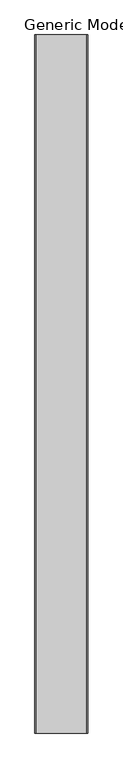
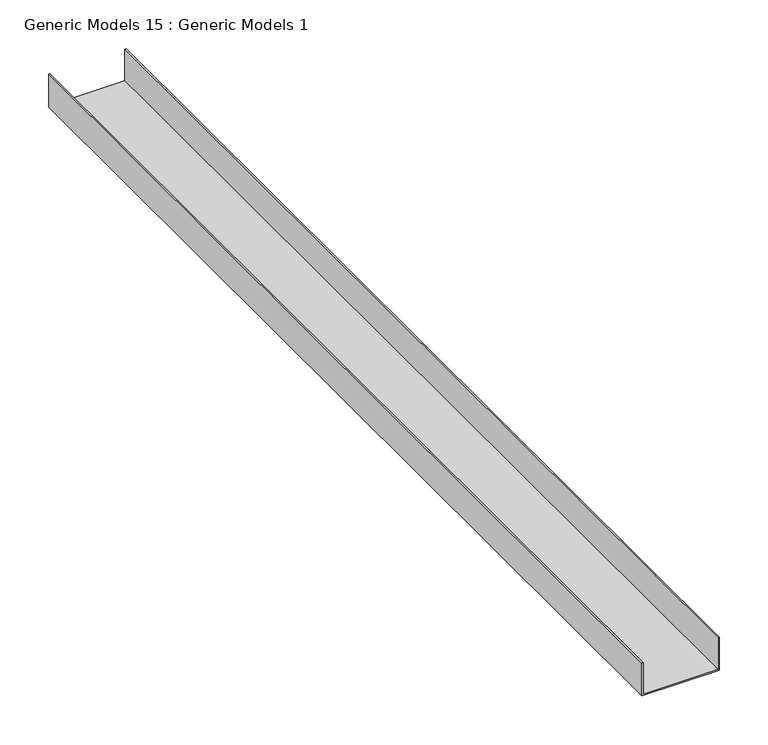
"""IFC4 building model written with IfcOpenShell, lengths in millimetres: proxy geometry, Generic Models 15 : Generic Models 1."""

from ifc_helpers import new_model, si_unit, frame, origin, place, context, project, spatial, polyline, outline, extrude, source, transform, mapped, element, save


def generic_models_15_generic_models_1_da732fbf(model_context):
    return source(origin(), model_context, "Body", "SweptSolid", [
        extrude(outline(polyline([(-1924.4473206, 52650.4446108), (-1883.1723206, 52650.4446108), (-1883.1723206, 52648.8571108), (-1922.8598206, 52648.8571108), (-1922.8598206, 52559.9571108), (-1883.1723206, 52559.9571108), (-1883.1723206, 52558.3696108), (-1924.4473206, 52558.3696108), (-1924.4473206, 52650.4446108)])), frame((0.0, 0.0, 0.0), z_axis=(0.0, 1.0, 0.0), x_axis=(0.0, 0.0, 1.0)), (0.0, 0.0, 1.0), 1219.2),
    ])


if __name__ == "__main__":
    model = new_model("IFC4")
    model_context = context("Model", 3, world=origin())
    ifc_project = project(units=[si_unit("LENGTHUNIT", "METRE", prefix="MILLI")], contexts=[model_context])
    site = spatial("IfcSite", under=ifc_project)
    building = spatial("IfcBuilding", under=site)
    placement = place(None, origin())
    generic_models_15_generic_models_1_shape = generic_models_15_generic_models_1_da732fbf(model_context)
    element("IfcBuildingElementProxy", 1, Name="Generic Models 15 : Generic Models 1", ObjectType="Generic Models 15 : Generic Models 1", at=placement, inside=building, context=model_context, shape_type="MappedRepresentation", body=[
        mapped(generic_models_15_generic_models_1_shape, transform((0.0, 0.0, 0.0), x_axis=(1.0, 0.0, 0.0), y_axis=(0.0, 1.0, 0.0), z_axis=(0.0, 0.0, 1.0))),
    ])
    save(model, "model.ifc")

# Revit data of these elements
# Element 1 (IfcBuildingElementProxy, "Generic Models 15 : Generic Models 1")
#   Materials on its faces: "METAL RUNNER CHANNEL; FASTEN @ 24\" O.C."
# Materials
#   "METAL RUNNER CHANNEL; FASTEN @ 24\" O.C.": class "Unassigned", colour RGB 210 209 208, transparency 0, Keynote = "M05121300.02", Cost = 0
